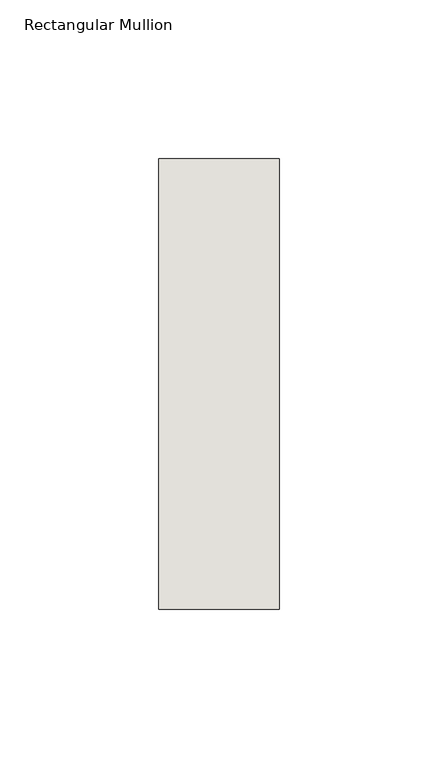
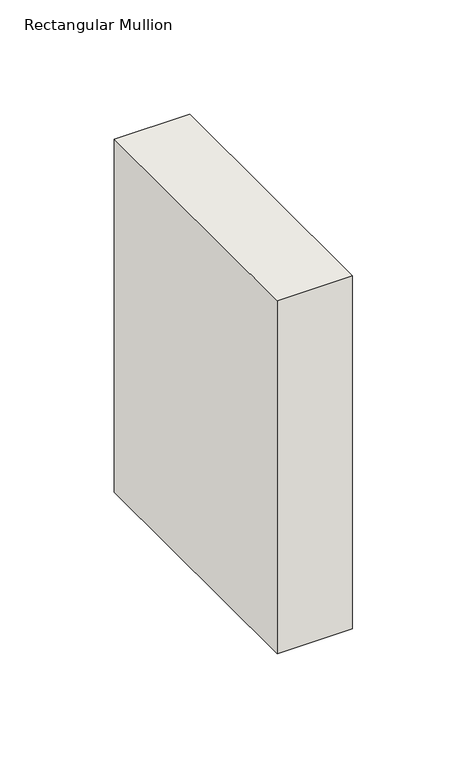
"""IFC4 building model written with IfcOpenShell, lengths in millimetres: wall geometry, Rectangular Mullion : NLRS_21_CWM_hsb-regel 38x142_gen_rsf."""

from ifc_helpers import new_model, si_unit, frame, origin, place, context, project, spatial, polyline, outline, extrude, source, transform, mapped, element, save


def rectangular_mullion_6dedba73(model_context):
    return source(origin(), model_context, "Body", "SweptSolid", [
        extrude(outline(polyline([(0.0, -71.0), (-38.0, -71.0), (-38.0, 71.0), (0.0, 71.0), (0.0, -71.0)])), frame((0.0, 0.0, -187.9999997), z_axis=(0.0, 0.0, 1.0), x_axis=(1.0, 0.0, 0.0)), (0.0, 0.0, 1.0), 187.9999997),
    ])


if __name__ == "__main__":
    model = new_model("IFC4")
    model_context = context("Model", 3, world=origin())
    ifc_project = project(units=[si_unit("LENGTHUNIT", "METRE", prefix="MILLI")], contexts=[model_context])
    site = spatial("IfcSite", under=ifc_project)
    building = spatial("IfcBuilding", under=site)
    placement = place(None, origin())
    rectangular_mullion_shape = rectangular_mullion_6dedba73(model_context)
    element("IfcWall", 1, ObjectType="Rectangular Mullion : NLRS_21_CWM_hsb-regel 38x142_gen_rsf", at=placement, inside=building, context=model_context, shape_type="MappedRepresentation", body=[
        mapped(rectangular_mullion_shape, transform((0.0, 0.0, 0.0), x_axis=(1.0, 0.0, 0.0), y_axis=(0.0, 1.0, 0.0), z_axis=(0.0, 0.0, 1.0))),
    ])
    save(model, "model.ifc")

# Revit data of these elements
# Type "Rectangular Mullion : NLRS_21_CWM_hsb-regel 38x142_gen_rsf"
#   Type IfcGUID = "07M7mRoiH1CR8m_RSKIwpF"
#   Assembly Code = "21.10"
#   IfcExportAs = "IfcWall"
#   built-in parameter 1007322 = 0.465879 (stored number, unit not read)
#   built-in parameter 1007321 = 0.062336 (stored number, unit not read)
#   built-in parameter 1007320 = 0.062336 (stored number, unit not read)
# Element 1 (IfcWall, "Rectangular Mullion : NLRS_21_CWM_hsb-regel 38x142_gen_rsf")
#   Materials on its faces: "NLRS_i2_hout naaldhout vuren_gen_rsf"
# Materials
#   "NLRS_i2_hout naaldhout vuren_gen_rsf": class "I - Hout", colour RGB 234 199 147, transparency 0, Keynote = "i2", Manufacturer = "Revit Standards Foundation", URL = "www.revitstandards.org", Description = "hout vuren", Cost = 0
